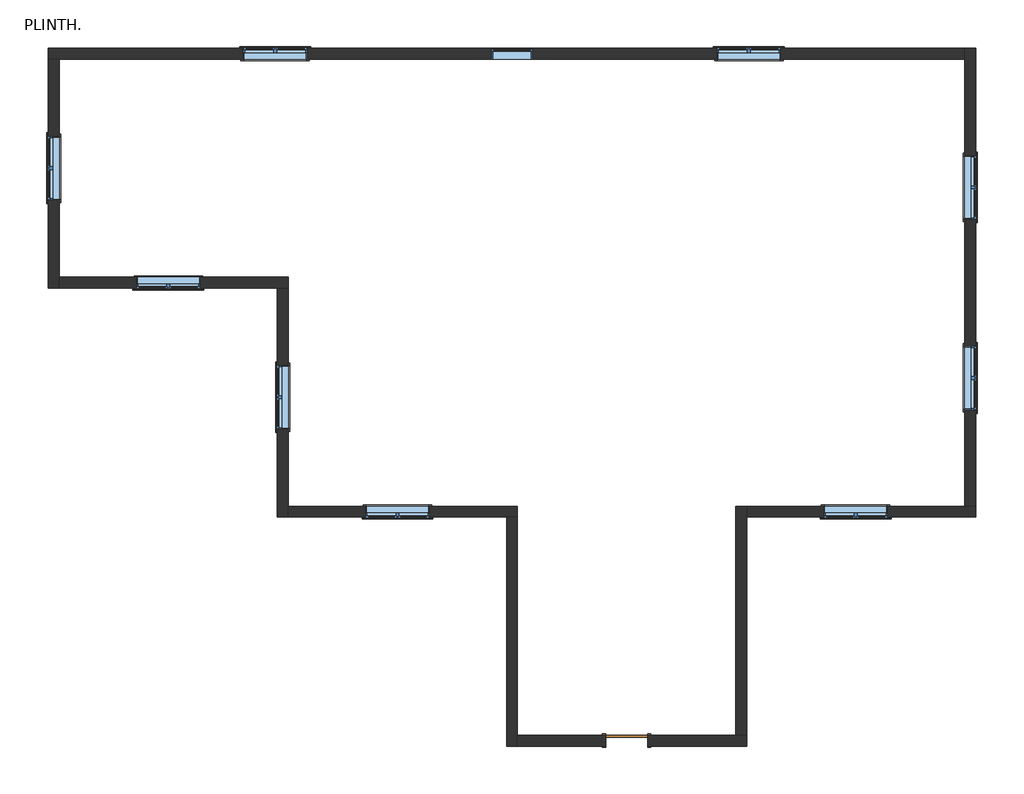
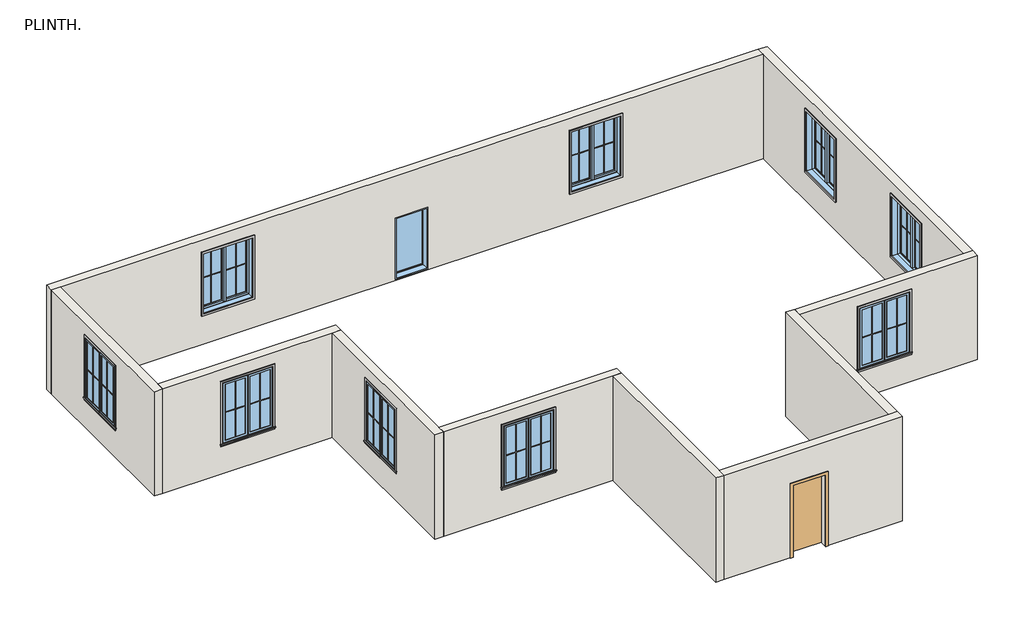
# One storey: 36 proxies, 10 walls, 10 windows, 1 door.
# Revit data of these elements (continued)
# Elements 1, 2, 3, 4, 5, 6, 7, 8, 9, 10, 11, 12, 13, 14, 15, 16, 17, 18 (IfcBuildingElementProxy, "M_Muntin Pattern_2x2 : M_Muntin Pattern_2x2")
#   Width = 56.3475 cm
#   Height = 166.03 cm
#   Interior Material = Wood - Stained
#   Exterior Material = Clad - White
#   Phase Created = New Construction
#   Materials on its faces: "Clad - White", "Wood - Stained"
# Elements 19, 20, 21, 22, 23, 24, 25, 26, 27 (IfcBuildingElementProxy, "M_Trim-Window-Exterior-Flat : with Sill")
#   Opening Width = 140 cm
#   Opening Height = 180 cm
#   Trim Material = Clad - White
#   Phase Created = New Construction
#   Materials on its faces: "Clad - White"
# Elements 28, 29, 30, 31, 32, 33, 34, 35, 36 (IfcBuildingElementProxy, "M_Trim-Window-Interior-Flat : Picture Frame")
#   Opening Width = 140 cm
#   Opening Height = 180 cm
#   Trim Material = Wood - Stained
#   Phase Created = New Construction
#   Materials on its faces: "Wood - Stained"
# Element 37 (IfcDoor, "M_Single-Flush : 0915 x 2134mm")
#   Phase Created = New Construction
#   Materials on its faces: "Door - Frame", "Door - Panel"
# Elements 38, 39, 40, 41, 42, 43, 44, 45, 46, 47 (IfcWall, "WALL24")
#   Top Offset = 0 cm
#   Base Offset = 0 cm
#   Unconnected Height = 310 cm
#   wall height = 310 cm
#   Phase Created = New Construction
#   Base Constraint = PLINTH.
#   Materials on its faces: "Default Wall"
# Element 48 (IfcWindow, "M_Fixed : 0915 x 1830mm")
#   Mark = "6"
#   Phase Created = New Construction
#   Materials on its faces: "Sash", "Glass"
# Element 49 (IfcWindow, "M_Window-Casement-Double : 1400 x 1800mm")
#   Mark = "1"
#   Window Inset = 0 cm
#   Interior Wall Closure = 5.475 cm
#   Frame Extension = 0.635 cm
#   Exterior Wall Closure = 3.18 cm
#   Interior Trim Visibility = yes
#   Exterior Trim Visibility = yes
#   Phase Created = New Construction
#   Materials on its faces: "Wood - Stained", "Glass", "Clad - White"
# Element 50 (IfcWindow, "M_Window-Casement-Double : 1400 x 1800mm")
#   Mark = "2"
#   Window Inset = 0 cm
#   Interior Wall Closure = 5.475 cm
#   Frame Extension = 0.635 cm
#   Exterior Wall Closure = 3.18 cm
#   Interior Trim Visibility = yes
#   Exterior Trim Visibility = yes
#   Phase Created = New Construction
#   Materials on its faces: "Wood - Stained", "Glass", "Clad - White"
# Element 51 (IfcWindow, "M_Window-Casement-Double : 1400 x 1800mm")
#   Mark = "3"
#   Window Inset = 0 cm
#   Interior Wall Closure = 5.475 cm
#   Frame Extension = 0.635 cm
#   Exterior Wall Closure = 3.18 cm
#   Interior Trim Visibility = yes
#   Exterior Trim Visibility = yes
#   Phase Created = New Construction
#   Materials on its faces: "Wood - Stained", "Glass", "Clad - White"
# Element 52 (IfcWindow, "M_Window-Casement-Double : 1400 x 1800mm")
#   Mark = "4"
#   Window Inset = 0 cm
#   Interior Wall Closure = 5.475 cm
#   Frame Extension = 0.635 cm
#   Exterior Wall Closure = 3.18 cm
#   Interior Trim Visibility = yes
#   Exterior Trim Visibility = yes
#   Phase Created = New Construction
#   Materials on its faces: "Wood - Stained", "Glass", "Clad - White"
# Element 53 (IfcWindow, "M_Window-Casement-Double : 1400 x 1800mm")
#   Mark = "5"
#   Window Inset = 0 cm
#   Interior Wall Closure = 5.475 cm
#   Frame Extension = 0.635 cm
#   Exterior Wall Closure = 3.18 cm
#   Interior Trim Visibility = yes
#   Exterior Trim Visibility = yes
#   Phase Created = New Construction
#   Materials on its faces: "Wood - Stained", "Glass", "Clad - White"
# Element 54 (IfcWindow, "M_Window-Casement-Double : 1400 x 1800mm")
#   Mark = "7"
#   Window Inset = 0 cm
#   Interior Wall Closure = 5.475 cm
#   Frame Extension = 0.635 cm
#   Exterior Wall Closure = 3.18 cm
#   Interior Trim Visibility = yes
#   Exterior Trim Visibility = yes
#   Phase Created = New Construction
#   Materials on its faces: "Wood - Stained", "Glass", "Clad - White"
# Element 55 (IfcWindow, "M_Window-Casement-Double : 1400 x 1800mm")
#   Mark = "8"
#   Window Inset = 0 cm
#   Interior Wall Closure = 5.475 cm
#   Frame Extension = 0.635 cm
#   Exterior Wall Closure = 3.18 cm
#   Interior Trim Visibility = yes
#   Exterior Trim Visibility = yes
#   Phase Created = New Construction
#   Materials on its faces: "Wood - Stained", "Glass", "Clad - White"
# Element 56 (IfcWindow, "M_Window-Casement-Double : 1400 x 1800mm")
#   Mark = "9"
#   Window Inset = 0 cm
#   Interior Wall Closure = 5.475 cm
#   Frame Extension = 0.635 cm
#   Exterior Wall Closure = 3.18 cm
#   Interior Trim Visibility = yes
#   Exterior Trim Visibility = yes
#   Phase Created = New Construction
#   Materials on its faces: "Wood - Stained", "Glass", "Clad - White"
# Element 57 (IfcWindow, "M_Window-Casement-Double : 1400 x 1800mm")
#   Mark = "10"
#   Window Inset = 0 cm
#   Interior Wall Closure = 5.475 cm
#   Frame Extension = 0.635 cm
#   Exterior Wall Closure = 3.18 cm
#   Interior Trim Visibility = yes
#   Exterior Trim Visibility = yes
#   Phase Created = New Construction
#   Materials on its faces: "Wood - Stained", "Glass", "Clad - White"
# Materials
#   "Door - Panel": class "Wood", colour RGB 210 159 95, transparency 0, Cost = 0
#   "Door - Frame": class "Miscellaneous", colour RGB 118 70 51, transparency 0, Cost = 0
#   "Sash": class "Wood", colour RGB 224 178 126, transparency 0, Cost = 0
#   "Glass": class "Glass", colour RGB 0 128 192, transparency 0.9, Description = "Soda Lime Glass", Cost = 0
#   "Wood - Stained": class "Wood", colour RGB 224 178 126, transparency 0, Cost = 0
#   "Clad - White": class "Wood", colour RGB 242 242 238, transparency 0, Cost = 0
#   "Default Wall": class "Miscellaneous", colour RGB 128 128 128, transparency 0, Cost = 0
